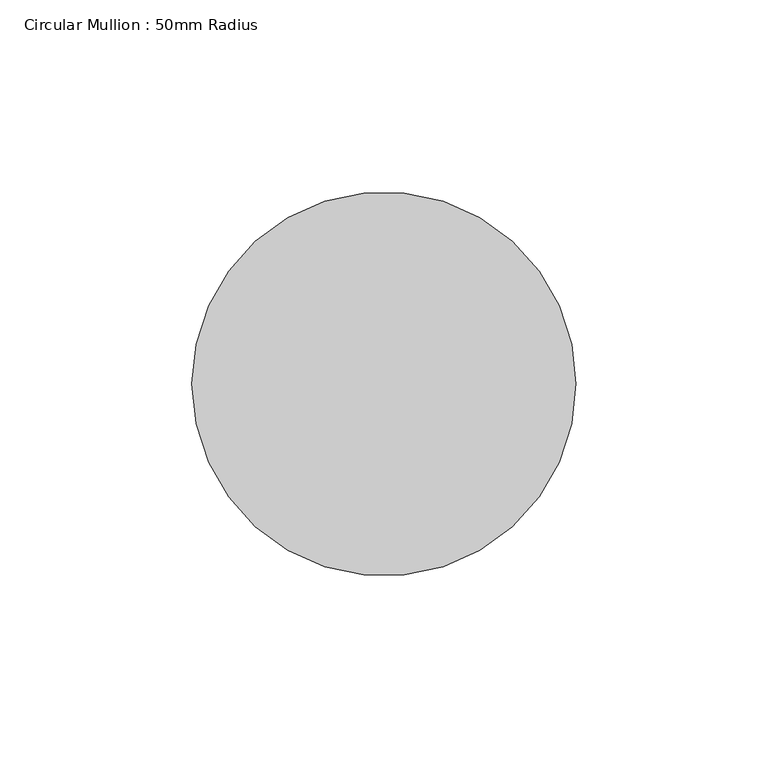
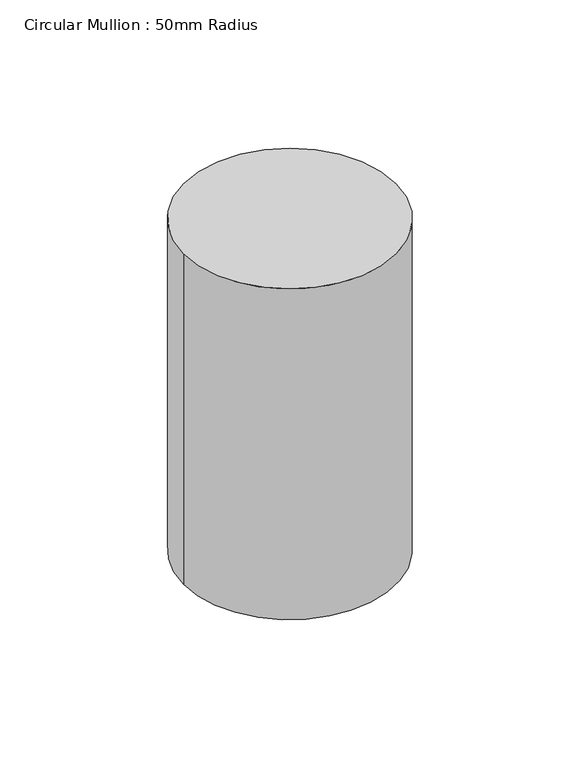
"""IFC4 building model written with IfcOpenShell, lengths in millimetres: member geometry, Circular Mullion : 50mm Radius."""

from ifc_helpers import new_model, si_unit, point, frame, origin, origin_2d, place, context, project, spatial, circle_curve, trimmed, segment, composite_curve, outline, extrude, source, transform, mapped, element, save


def circular_mullion_50mm_radius_ec6fe9e2(model_context):
    return source(origin(), model_context, "Body", "SweptSolid", [
        extrude(outline(composite_curve([segment(trimmed(circle_curve(origin_2d(), 50.0), [point((50.0, 0.0))], [point((-50.0, 0.0))], False, "CARTESIAN"), True, "CONTINUOUS"), segment(trimmed(circle_curve(origin_2d(), 50.0), [point((-50.0, 0.0))], [point((50.0, 0.0))], False, "CARTESIAN"), True, "CONTINUOUS")], self_intersect=False)), frame((0.0, 0.0, -164.6139612), z_axis=(0.0, 0.0, 1.0), x_axis=(1.0, 0.0, 0.0)), (0.0, 0.0, 1.0), 164.6139612),
    ])


if __name__ == "__main__":
    model = new_model("IFC4")
    model_context = context("Model", 3, world=origin())
    ifc_project = project(units=[si_unit("LENGTHUNIT", "METRE", prefix="MILLI")], contexts=[model_context])
    site = spatial("IfcSite", under=ifc_project)
    building = spatial("IfcBuilding", under=site)
    placement = place(None, origin())
    circular_mullion_50mm_radius_shape = circular_mullion_50mm_radius_ec6fe9e2(model_context)
    element("IfcMember", 1, ObjectType="Circular Mullion : 50mm Radius", at=placement, inside=building, context=model_context, shape_type="MappedRepresentation", body=[
        mapped(circular_mullion_50mm_radius_shape, transform((0.0, 0.0, 0.0), x_axis=(1.0, 0.0, 0.0), y_axis=(0.0, 1.0, 0.0), z_axis=(0.0, 0.0, 1.0))),
    ])
    save(model, "model.ifc")

# Revit data of these elements
# Type "Circular Mullion : 50mm Radius"
#   built-in parameter 1007350 = 0.164042 (stored number, unit not read)
# Element 1 (IfcMember, "Circular Mullion : 50mm Radius")
#   Materials on its faces: "Aluminium"
# Materials
#   "Aluminium": class "Metal", colour RGB 247 247 247, transparency 0, Description = "Aluminium 6061", Cost = 0
